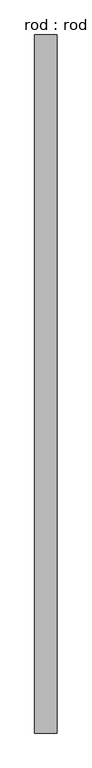
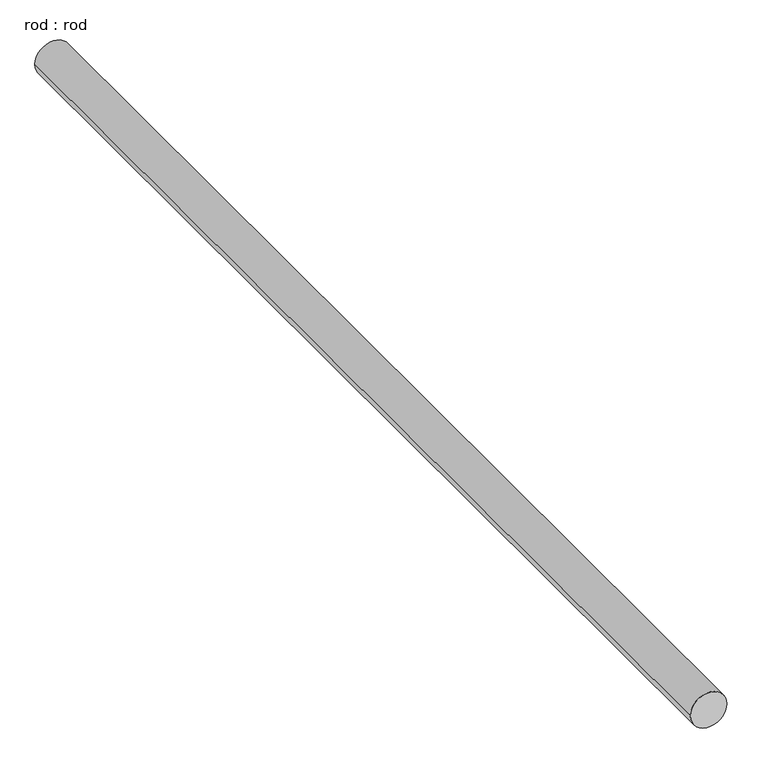
"""IFC4 building model written with IfcOpenShell, lengths in millimetres: proxy geometry, rod : rod."""

from ifc_helpers import new_model, si_unit, point, frame, frame_2d, origin, place, context, project, spatial, circle_curve, trimmed, segment, composite_curve, outline, extrude, source, transform, mapped, element, save


def rod_rod_2d6b6431(model_context):
    return source(origin(), model_context, "Body", "SweptSolid", [
        extrude(outline(composite_curve([segment(trimmed(circle_curve(frame_2d((0.0108462, 0.0)), 200.0), [point((0.0108462, 200.0))], [point((0.0108462, -200.0))], False, "CARTESIAN"), True, "CONTINUOUS"), segment(trimmed(circle_curve(frame_2d((0.0108462, 0.0)), 200.0), [point((0.0108462, -200.0))], [point((0.0108462, 200.0))], False, "CARTESIAN"), True, "CONTINUOUS")], self_intersect=False)), frame((0.0, -2129.4936069, 0.0), z_axis=(0.0, 1.0, 0.0), x_axis=(0.0, 0.0, 1.0)), (0.0, 0.0, 1.0), 12444.4444444),
    ])


if __name__ == "__main__":
    model = new_model("IFC4")
    model_context = context("Model", 3, world=origin())
    ifc_project = project(units=[si_unit("LENGTHUNIT", "METRE", prefix="MILLI")], contexts=[model_context])
    site = spatial("IfcSite", under=ifc_project)
    building = spatial("IfcBuilding", under=site)
    placement = place(None, origin())
    rod_rod_shape = rod_rod_2d6b6431(model_context)
    element("IfcBuildingElementProxy", 1, Name="rod : rod", ObjectType="rod : rod", at=placement, inside=building, context=model_context, shape_type="MappedRepresentation", body=[
        mapped(rod_rod_shape, transform((0.0, 0.0, 0.0), x_axis=(1.0, 0.0, 0.0), y_axis=(0.0, 1.0, 0.0), z_axis=(0.0, 0.0, 1.0))),
    ])
    save(model, "model.ifc")

# Revit data of these elements
# Type "rod : rod"
#   Default Elevation = 0
